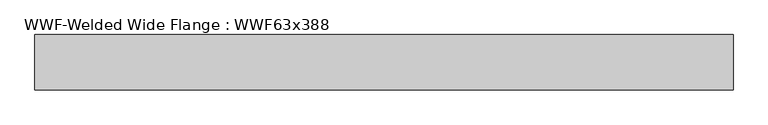
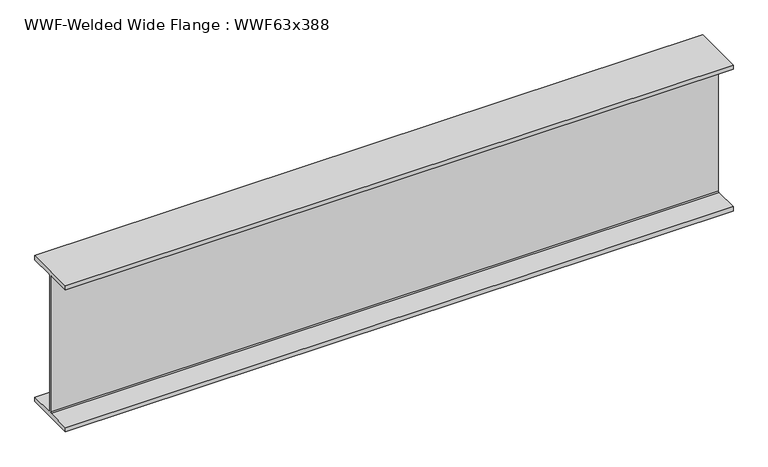
"""IFC4 building model written with IfcOpenShell, lengths in millimetres: beam geometry, WWF-Welded Wide Flange : WWF63x388."""

import ifcopenshell
import ifcopenshell.guid

model = None  # the IFC model being written
_history = None  # IfcOwnerHistory: only IFC2X3 demands one
_inside = {}  # id of a spatial element -> (the spatial element, [elements in it])
_under = {}  # id of a project, library or spatial element -> (it, [spatial elements below it])
_declared = {}  # id of a project -> (the project, [libraries it declares])
_typed = {}  # id of a type object -> (the type object, [elements of that type])
_made_of = {}  # id of a material, layer set ... -> (it, [elements and type objects made of it])


def new_model(schema):
    """Start an empty IFC model of exactly this schema.

    Asked for "IFC4X3", IfcOpenShell would pick the latest addendum, in which some entities
    have other attributes; the version numbers below select the first issue.
    IFC2X3 requires an IfcOwnerHistory on every rooted entity: one is made here for all.
    """
    global model, _history
    if schema == "IFC4X3":
        model = ifcopenshell.file(schema_version=(4, 3, 0, 0))
    else:
        model = ifcopenshell.file(schema=schema)
    _inside.clear()
    _under.clear()
    _declared.clear()
    _typed.clear()
    _made_of.clear()
    _history = None
    if model.schema == "IFC2X3":
        org = make("IfcOrganization", Name="unknown")
        user = make(
            "IfcPersonAndOrganization",
            ThePerson=make("IfcPerson", FamilyName="unknown"),
            TheOrganization=org,
        )
        app = make(
            "IfcApplication",
            ApplicationDeveloper=org,
            Version="unknown",
            ApplicationFullName="unknown",
            ApplicationIdentifier="unknown",
        )
        _history = make(
            "IfcOwnerHistory",
            OwningUser=user,
            OwningApplication=app,
            ChangeAction="ADDED",
            CreationDate=0,
        )
    return model


def make(cls, **values):
    """One entity of the class cls with the attributes given. An attribute that is None is left unset."""
    return model.create_entity(
        cls, **{name: value for name, value in values.items() if value is not None}
    )


def rooted(cls, **values):
    """An entity with a GlobalId (a new one), such as an element, a storey or a relation."""
    return make(cls, GlobalId=ifcopenshell.guid.new(), OwnerHistory=_history, **values)


def si_unit(unit_type, name, prefix=None):
    """IfcSIUnit, for example si_unit("LENGTHUNIT", "METRE", prefix="MILLI")."""
    return make("IfcSIUnit", UnitType=unit_type, Prefix=prefix, Name=name)


def assignment(units):
    """IfcUnitAssignment: the units of a project."""
    return None if units is None else make("IfcUnitAssignment", Units=units)


def point(xyz):
    """IfcCartesianPoint."""
    return None if xyz is None else make("IfcCartesianPoint", Coordinates=xyz)


def direction(xyz):
    """IfcDirection."""
    return None if xyz is None else make("IfcDirection", DirectionRatios=xyz)


def frame(location, z_axis=None, x_axis=None):
    """IfcAxis2Placement3D, a coordinate frame: its origin and axes. An axis left out is left unset."""
    return make(
        "IfcAxis2Placement3D",
        Location=point(location),
        Axis=direction(z_axis),
        RefDirection=direction(x_axis),
    )


def origin():
    """The frame at (0, 0, 0) with its axes left unset."""
    return frame((0.0, 0.0, 0.0))


def place(relative_to, where):
    """IfcLocalPlacement: puts the frame where relative to a parent placement (None: the world)."""
    return make(
        "IfcLocalPlacement", PlacementRelTo=relative_to, RelativePlacement=where
    )


def context(
    kind, dimensions, precision=None, world=None, true_north=None, identifier=None
):
    """IfcGeometricRepresentationContext, for example the 3D "Model" context."""
    return make(
        "IfcGeometricRepresentationContext",
        ContextIdentifier=identifier,
        ContextType=kind,
        CoordinateSpaceDimension=dimensions,
        Precision=precision,
        WorldCoordinateSystem=world,
        TrueNorth=true_north,
    )


def project(units=None, contexts=None):
    """IfcProject with its units and contexts."""
    return rooted(
        "IfcProject",
        Name="project",
        RepresentationContexts=contexts,
        UnitsInContext=assignment(units),
    )


def spatial(cls, under=None, at=None, **own):
    """A site, building, storey or space (cls), placed at a placement, below another one or the project."""
    s = rooted(cls, ObjectPlacement=at, **own)
    if under is not None:
        _under.setdefault(under.id(), (under, []))[1].append(s)
    return s


def polyline(points):
    """IfcPolyline through the points."""
    return make("IfcPolyline", Points=[point(p) for p in points])


def outline(outer, holes=None, kind="AREA"):
    """IfcArbitraryClosedProfileDef: a profile drawn as a closed curve; with holes, ...WithVoids."""
    if holes is None:
        return make("IfcArbitraryClosedProfileDef", ProfileType=kind, OuterCurve=outer)
    return make(
        "IfcArbitraryProfileDefWithVoids",
        ProfileType=kind,
        OuterCurve=outer,
        InnerCurves=holes,
    )


def extrude(swept, where, along, depth):
    """IfcExtrudedAreaSolid: the profile swept, set in the frame where, extruded along a direction by depth."""
    return make(
        "IfcExtrudedAreaSolid",
        SweptArea=swept,
        Position=where,
        ExtrudedDirection=direction(along),
        Depth=depth,
    )


def shape(context_of_items, identifier, shape_type, items):
    """IfcShapeRepresentation: the items that make up one representation, for example the "Body"."""
    return make(
        "IfcShapeRepresentation",
        ContextOfItems=context_of_items,
        RepresentationIdentifier=identifier,
        RepresentationType=shape_type,
        Items=items,
    )


def source(mapping_origin, context_of_items, identifier, shape_type, items):
    """IfcRepresentationMap: a shape defined once, which mapped items show again and again."""
    return make(
        "IfcRepresentationMap",
        MappingOrigin=mapping_origin,
        MappedRepresentation=shape(context_of_items, identifier, shape_type, items),
    )


def transform(
    local_origin,
    x_axis=None,
    y_axis=None,
    z_axis=None,
    scale=None,
    scale2=None,
    scale3=None,
    uniform=True,
):
    """IfcCartesianTransformationOperator3D, or its non-uniform kind. x_axis, y_axis, z_axis: its Axis1, 2, 3."""
    if uniform:
        return make(
            "IfcCartesianTransformationOperator3D",
            Axis1=direction(x_axis),
            Axis2=direction(y_axis),
            LocalOrigin=point(local_origin),
            Scale=scale,
            Axis3=direction(z_axis),
        )
    return make(
        "IfcCartesianTransformationOperator3DnonUniform",
        Axis1=direction(x_axis),
        Axis2=direction(y_axis),
        LocalOrigin=point(local_origin),
        Scale=scale,
        Axis3=direction(z_axis),
        Scale2=scale2,
        Scale3=scale3,
    )


def mapped(mapping_source, mapping_target):
    """IfcMappedItem: shows the shape of a source again, moved by a transform."""
    return make(
        "IfcMappedItem", MappingSource=mapping_source, MappingTarget=mapping_target
    )


def made_of(thing, what):
    """Note that an element or type object is made of a material, layer set ...; save() writes the relation."""
    if what is not None:
        _made_of.setdefault(what.id(), (what, []))[1].append(thing)
    return thing


def element(
    cls,
    number,
    at=None,
    inside=None,
    cuts=None,
    type_object=None,
    material=None,
    context=None,
    identifier="Body",
    shape_type=None,
    held_by="IfcProductDefinitionShape",
    body=None,
    shapes=None,
    **own,
):
    """One element of the class cls, such as IfcWall. Its Tag is "e" and its number.

    at: its placement. inside: the storey or other place that contains it. cuts: it is an
    opening in that element (IfcRelVoidsElement). A single representation is given by context,
    identifier, shape_type and body (its items); several are given by shapes. held_by: the class
    of the entity that holds the representations. save() writes the other relations.
    """
    e = rooted(cls, Tag="e%d" % number, ObjectPlacement=at, **own)
    if body is not None:
        shapes = [shape(context, identifier, shape_type, body)]
    if shapes is not None:
        e.Representation = make(held_by, Representations=shapes)
    if inside is not None:
        _inside.setdefault(inside.id(), (inside, []))[1].append(e)
    if cuts is not None:
        rooted(
            "IfcRelVoidsElement", RelatingBuildingElement=cuts, RelatedOpeningElement=e
        )
    if type_object is not None:
        _typed.setdefault(type_object.id(), (type_object, []))[1].append(e)
    return made_of(e, material)


def aggregate(whole, parts):
    """IfcRelAggregates: a whole, such as a stair, and the parts it consists of."""
    return rooted("IfcRelAggregates", RelatingObject=whole, RelatedObjects=parts)


def save(model, path):
    """Write the relations noted so far, then the file.

    IfcRelAggregates (storeys below a building ...), IfcRelContainedInSpatialStructure (elements
    in a storey), IfcRelDefinesByType, IfcRelAssociatesMaterial and IfcRelDeclares: one each for
    every whole, place, type object, material and project.
    """
    for whole, parts in _under.values():
        aggregate(whole, parts)
    for where, things in _inside.values():
        rooted(
            "IfcRelContainedInSpatialStructure",
            RelatedElements=things,
            RelatingStructure=where,
        )
    for kind, things in _typed.values():
        rooted("IfcRelDefinesByType", RelatedObjects=things, RelatingType=kind)
    for what, things in _made_of.values():
        rooted("IfcRelAssociatesMaterial", RelatedObjects=things, RelatingMaterial=what)
    for by, libraries in _declared.values():
        rooted("IfcRelDeclares", RelatingContext=by, RelatedDefinitions=libraries)
    model.write(path)


def wwf_welded_wide_flange_wwf63x388_c82ffaba(model_context):
    return source(origin(), model_context, "Body", "SweptSolid", [
        extrude(outline(polyline([(274.955, -755.015), (274.955, -799.973), (-274.955, -799.973), (-274.955, -755.015), (-19.05, -755.015), (-8.001, -743.966), (-8.001, 743.966), (-19.05, 755.015), (-274.955, 755.015), (-274.955, 799.973), (274.955, 799.973), (274.955, 755.015), (19.05, 755.015), (8.001, 743.966), (8.001, -743.966), (19.05, -755.015), (274.955, -755.015)])), frame((-3184.5821682, 0.0, 0.0), z_axis=(1.0, 0.0, 0.0), x_axis=(0.0, 1.0, 0.0)), (0.0, 0.0, 1.0), 6931.7444444),
    ])


if __name__ == "__main__":
    model = new_model("IFC4")
    model_context = context("Model", 3, world=origin())
    ifc_project = project(units=[si_unit("LENGTHUNIT", "METRE", prefix="MILLI")], contexts=[model_context])
    site = spatial("IfcSite", under=ifc_project)
    building = spatial("IfcBuilding", under=site)
    placement = place(None, origin())
    wwf_welded_wide_flange_wwf63x388_shape = wwf_welded_wide_flange_wwf63x388_c82ffaba(model_context)
    element("IfcBeam", 1, ObjectType="WWF-Welded Wide Flange : WWF63x388", at=placement, inside=building, context=model_context, shape_type="MappedRepresentation", body=[
        mapped(wwf_welded_wide_flange_wwf63x388_shape, transform((0.0, 0.0, 0.0), x_axis=(1.0, 0.0, 0.0), y_axis=(0.0, 1.0, 0.0), z_axis=(0.0, 0.0, 1.0))),
    ])
    save(model, "model.ifc")

# Revit data of these elements
# Type "WWF-Welded Wide Flange : WWF63x388"
#   Assembly Code = "B10"
#   Nominal d = "12"
#   W = 388
#   Length [instance default] = 1524 mm
#   bf = 549.91 mm
#   d = 1599.946 mm
#   k = 19.05 mm
#   tf = 44.958 mm
#   tw = 16.002 mm
#   A = 0.0735482 m²
#   Structural Material [instance default] = Steel ASTM A572
# Element 1 (IfcBeam, "WWF-Welded Wide Flange : WWF63x388")
#   Structural Material = Metal - Steel 43-275
#   Materials on its faces: "Metal - Steel 43-275"
# Materials
#   "Steel ASTM A572": class "Metal", colour RGB 247 247 247, transparency 0, Description = "Structural steel, high strength low alloy, ASTM - A572 - 50", Cost = 0
#   "Metal - Steel 43-275": class "Metal", colour RGB 247 247 247, transparency 0, Cost = 0
